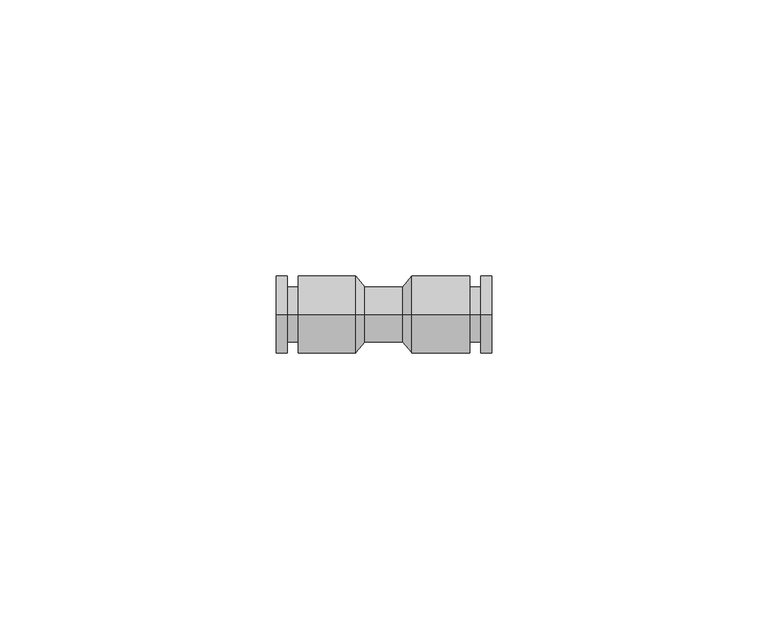
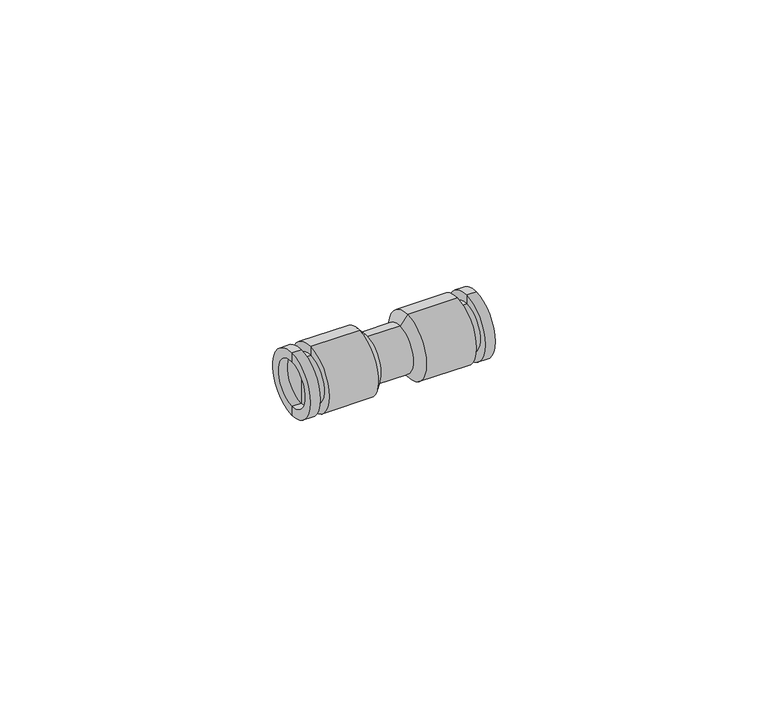
"""IFC4 building model written with IfcOpenShell, lengths in millimetres: proxy geometry, ➾ Фитинг прямой : ➾ Фитинг прямой."""

from ifc_helpers import new_model, si_unit, frame, origin, place, context, project, spatial, polyline, circle_curve, source, transform, mapped, element, save
from ifc_brep_helpers import plane_surface, cylinder_surface, revolved_surface, advanced_brep


def specialty_equipment_034aae71(model_context):
    return source(origin(), model_context, "Body", "AdvancedBrep", [
        advanced_brep(
        [(2.0, 0.0, -5.0), (2.0, 0.0, 5.0), (3.9823242, 0.0, 5.0), (3.9823242, 0.0, -5.0), (2.0, 0.0, 0.0), (37.0, 0.0, -5.0), (37.0, 0.0, 5.0), (37.0, 0.0, 0.0), (35.0176758, 0.0, -5.0), (35.0176758, 0.0, 5.0), (35.0176758, 0.0, -6.9783313), (35.0176758, 0.0, 6.9783313), (24.5665024, 0.0, -6.9783313), (24.5665024, 0.0, 6.9783313), (22.9064853, 0.0, -5.0), (22.9064853, 0.0, 5.0), (16.034289, 0.0, -5.0), (16.034289, 0.0, 5.0), (14.3742719, 0.0, -6.9783313), (14.3742719, 0.0, 6.9783313), (3.9823242, 0.0, -6.9783313), (3.9823242, 0.0, 6.9783313)],
        [
            (0, 1, circle_curve(frame((2.0, 0.0, 0.0), z_axis=(1.0, 0.0, 0.0), x_axis=(0.0, 0.0, 1.0)), 5.0)),
            (1, 2),
            (2, 3, circle_curve(frame((3.9823242, 0.0, 0.0), z_axis=(-1.0, 0.0, 0.0), x_axis=(0.0, 0.0, 1.0)), 5.0)),
            (3, 0),
            (1, 0, circle_curve(frame((2.0, 0.0, 0.0), z_axis=(1.0, 0.0, 0.0), x_axis=(0.0, 0.0, 1.0)), 5.0)),
            (3, 2, circle_curve(frame((3.9823242, 0.0, 0.0), z_axis=(-1.0, 0.0, 0.0), x_axis=(0.0, 0.0, 1.0)), 5.0)),
            (4, 1),
            (0, 4),
            (5, 6, circle_curve(frame((37.0, 0.0, 0.0), z_axis=(1.0, 0.0, 0.0), x_axis=(0.0, 0.0, 1.0)), 5.0)),
            (6, 7),
            (7, 5),
            (6, 5, circle_curve(frame((37.0, 0.0, 0.0), z_axis=(1.0, 0.0, 0.0), x_axis=(0.0, 0.0, 1.0)), 5.0)),
            (8, 9, circle_curve(frame((35.0176758, 0.0, 0.0), z_axis=(1.0, 0.0, 0.0), x_axis=(0.0, 0.0, 1.0)), 5.0)),
            (9, 6),
            (5, 8),
            (9, 8, circle_curve(frame((35.0176758, 0.0, 0.0), z_axis=(1.0, 0.0, 0.0), x_axis=(0.0, 0.0, 1.0)), 5.0)),
            (10, 11, circle_curve(frame((35.0176758, 0.0, 0.0), z_axis=(1.0, 0.0, 0.0), x_axis=(0.0, 0.0, 1.0)), 6.9783313)),
            (11, 9),
            (8, 10),
            (11, 10, circle_curve(frame((35.0176758, 0.0, 0.0), z_axis=(1.0, 0.0, 0.0), x_axis=(0.0, 0.0, 1.0)), 6.9783313)),
            (12, 13, circle_curve(frame((24.5665024, 0.0, 0.0), z_axis=(1.0, 0.0, 0.0), x_axis=(0.0, 0.0, 1.0)), 6.9783313)),
            (13, 11),
            (10, 12),
            (13, 12, circle_curve(frame((24.5665024, 0.0, 0.0), z_axis=(1.0, 0.0, 0.0), x_axis=(0.0, 0.0, 1.0)), 6.9783313)),
            (14, 15, circle_curve(frame((22.9064853, 0.0, 0.0), z_axis=(1.0, 0.0, 0.0), x_axis=(0.0, 0.0, 1.0)), 5.0)),
            (15, 13),
            (12, 14),
            (15, 14, circle_curve(frame((22.9064853, 0.0, 0.0), z_axis=(1.0, 0.0, 0.0), x_axis=(0.0, 0.0, 1.0)), 5.0)),
            (16, 17, circle_curve(frame((16.034289, 0.0, 0.0), z_axis=(1.0, 0.0, 0.0), x_axis=(0.0, 0.0, 1.0)), 5.0)),
            (17, 15),
            (14, 16),
            (17, 16, circle_curve(frame((16.034289, 0.0, 0.0), z_axis=(1.0, 0.0, 0.0), x_axis=(0.0, 0.0, 1.0)), 5.0)),
            (18, 19, circle_curve(frame((14.3742719, 0.0, 0.0), z_axis=(1.0, 0.0, 0.0), x_axis=(0.0, 0.0, 1.0)), 6.9783313)),
            (19, 17),
            (16, 18),
            (19, 18, circle_curve(frame((14.3742719, 0.0, 0.0), z_axis=(1.0, 0.0, 0.0), x_axis=(0.0, 0.0, 1.0)), 6.9783313)),
            (20, 21, circle_curve(frame((3.9823242, 0.0, 0.0), z_axis=(1.0, 0.0, 0.0), x_axis=(0.0, 0.0, 1.0)), 6.9783313)),
            (21, 19),
            (18, 20),
            (21, 20, circle_curve(frame((3.9823242, 0.0, 0.0), z_axis=(1.0, 0.0, 0.0), x_axis=(0.0, 0.0, 1.0)), 6.9783313)),
            (2, 21),
            (20, 3),
        ],
        [
            cylinder_surface(frame((-1506.5299635, 0.0, 0.0), z_axis=(-1.0, 0.0, 0.0), x_axis=(0.0, 0.0, 1.0)), 5.0),
            plane_surface(frame((2.0, 0.0, 0.0), z_axis=(-1.0, 0.0, 0.0), x_axis=(0.0, 0.0, 1.0))),
            plane_surface(frame((37.0, 0.0, 0.0), z_axis=(1.0, 0.0, 0.0), x_axis=(0.0, 0.0, 1.0))),
            plane_surface(frame((35.0176758, 0.0, 0.0), z_axis=(1.0, 0.0, 0.0), x_axis=(0.0, 0.0, 1.0))),
            cylinder_surface(frame((-1506.5299635, 0.0, 0.0), z_axis=(-1.0, 0.0, 0.0), x_axis=(0.0, 0.0, 1.0)), 6.9783313),
            revolved_surface(polyline([(24.5665024, 0.0, 6.9783313), (22.9064853, 0.0, 5.0)]), (-1506.5299635, 0.0, 0.0), (-1.0, 0.0, 0.0)),
            revolved_surface(polyline([(16.034289, 0.0, 5.0), (14.3742719, 0.0, 6.9783313)]), (-1506.5299635, 0.0, 0.0), (-1.0, 0.0, 0.0)),
            plane_surface(frame((3.9823242, 0.0, 0.0), z_axis=(-1.0, 0.0, 0.0), x_axis=(0.0, 0.0, 1.0))),
        ],
        [
            (0, [[1, 2, 3, 4]]),
            (0, [[5, -4, 6, -2]]),
            (1, [[7, -1, 8]]),
            (1, [[-8, -5, -7]]),
            (2, [[9, 10, 11]]),
            (2, [[12, -11, -10]]),
            (0, [[13, 14, -9, 15]]),
            (0, [[16, -15, -12, -14]]),
            (3, [[17, 18, -13, 19]]),
            (3, [[20, -19, -16, -18]]),
            (4, [[21, 22, -17, 23]]),
            (4, [[24, -23, -20, -22]]),
            (5, [[25, 26, -21, 27]]),
            (5, [[28, -27, -24, -26]]),
            (0, [[29, 30, -25, 31]]),
            (0, [[32, -31, -28, -30]]),
            (6, [[33, 34, -29, 35]]),
            (6, [[36, -35, -32, -34]]),
            (4, [[37, 38, -33, 39]]),
            (4, [[40, -39, -36, -38]]),
            (7, [[-3, 41, -37, 42]]),
            (7, [[-6, -42, -40, -41]]),
        ],
    ),
        advanced_brep(
        [(39.0, 0.0, -6.9783313), (39.0, 0.0, 6.9783313), (39.0, 0.0, 5.0), (39.0, 0.0, -5.0), (37.0, 0.0, -6.9783313), (37.0, 0.0, 6.9783313), (37.0, 0.0, -5.0), (37.0, 0.0, 5.0)],
        [
            (0, 1, circle_curve(frame((39.0, 0.0, 0.0), z_axis=(1.0, 0.0, 0.0), x_axis=(0.0, 0.0, 1.0)), 6.9783313)),
            (1, 2),
            (2, 3, circle_curve(frame((39.0, 0.0, 0.0), z_axis=(-1.0, 0.0, 0.0), x_axis=(0.0, 0.0, 1.0)), 5.0)),
            (3, 0),
            (1, 0, circle_curve(frame((39.0, 0.0, 0.0), z_axis=(1.0, 0.0, 0.0), x_axis=(0.0, 0.0, 1.0)), 6.9783313)),
            (3, 2, circle_curve(frame((39.0, 0.0, 0.0), z_axis=(-1.0, 0.0, 0.0), x_axis=(0.0, 0.0, 1.0)), 5.0)),
            (4, 5, circle_curve(frame((37.0, 0.0, 0.0), z_axis=(1.0, 0.0, 0.0), x_axis=(0.0, 0.0, 1.0)), 6.9783313)),
            (5, 1),
            (0, 4),
            (5, 4, circle_curve(frame((37.0, 0.0, 0.0), z_axis=(1.0, 0.0, 0.0), x_axis=(0.0, 0.0, 1.0)), 6.9783313)),
            (6, 7, circle_curve(frame((37.0, 0.0, 0.0), z_axis=(1.0, 0.0, 0.0), x_axis=(0.0, 0.0, 1.0)), 5.0)),
            (7, 5),
            (4, 6),
            (7, 6, circle_curve(frame((37.0, 0.0, 0.0), z_axis=(1.0, 0.0, 0.0), x_axis=(0.0, 0.0, 1.0)), 5.0)),
            (2, 7),
            (6, 3),
        ],
        [
            plane_surface(frame((39.0, 0.0, 0.0), z_axis=(1.0, 0.0, 0.0), x_axis=(0.0, 0.0, 1.0))),
            cylinder_surface(frame((-1469.5299635, 0.0, 0.0), z_axis=(-1.0, 0.0, 0.0), x_axis=(0.0, 0.0, 1.0)), 6.9783313),
            plane_surface(frame((37.0, 0.0, 0.0), z_axis=(-1.0, 0.0, 0.0), x_axis=(0.0, 0.0, 1.0))),
            revolved_surface(polyline([(37.0, 0.0, 5.0), (39.0, 0.0, 5.0)]), (-1469.5299635, 0.0, 0.0), (-1.0, 0.0, 0.0)),
        ],
        [
            (0, [[1, 2, 3, 4]]),
            (0, [[5, -4, 6, -2]]),
            (1, [[7, 8, -1, 9]]),
            (1, [[10, -9, -5, -8]]),
            (2, [[11, 12, -7, 13]]),
            (2, [[14, -13, -10, -12]]),
            (3, [[-3, 15, -11, 16]]),
            (3, [[-6, -16, -14, -15]]),
        ],
    ),
        advanced_brep(
        [(2.0, 0.0, -6.9783313), (2.0, 0.0, 6.9783313), (2.0, 0.0, 5.0), (2.0, 0.0, -5.0), (0.0, 0.0, -6.9783313), (0.0, 0.0, 6.9783313), (0.0, 0.0, -5.0), (0.0, 0.0, 5.0)],
        [
            (0, 1, circle_curve(frame((2.0, 0.0, 0.0), z_axis=(1.0, 0.0, 0.0), x_axis=(0.0, 0.0, 1.0)), 6.9783313)),
            (1, 2),
            (2, 3, circle_curve(frame((2.0, 0.0, 0.0), z_axis=(-1.0, 0.0, 0.0), x_axis=(0.0, 0.0, 1.0)), 5.0)),
            (3, 0),
            (1, 0, circle_curve(frame((2.0, 0.0, 0.0), z_axis=(1.0, 0.0, 0.0), x_axis=(0.0, 0.0, 1.0)), 6.9783313)),
            (3, 2, circle_curve(frame((2.0, 0.0, 0.0), z_axis=(-1.0, 0.0, 0.0), x_axis=(0.0, 0.0, 1.0)), 5.0)),
            (4, 5, circle_curve(frame((0.0, 0.0, 0.0), z_axis=(1.0, 0.0, 0.0), x_axis=(0.0, 0.0, 1.0)), 6.9783313)),
            (5, 1),
            (0, 4),
            (5, 4, circle_curve(frame((0.0, 0.0, 0.0), z_axis=(1.0, 0.0, 0.0), x_axis=(0.0, 0.0, 1.0)), 6.9783313)),
            (6, 7, circle_curve(frame((0.0, 0.0, 0.0), z_axis=(1.0, 0.0, 0.0), x_axis=(0.0, 0.0, 1.0)), 5.0)),
            (7, 5),
            (4, 6),
            (7, 6, circle_curve(frame((0.0, 0.0, 0.0), z_axis=(1.0, 0.0, 0.0), x_axis=(0.0, 0.0, 1.0)), 5.0)),
            (2, 7),
            (6, 3),
        ],
        [
            plane_surface(frame((2.0, 0.0, 0.0), z_axis=(1.0, 0.0, 0.0), x_axis=(0.0, 0.0, 1.0))),
            cylinder_surface(frame((-1506.5299635, 0.0, 0.0), z_axis=(-1.0, 0.0, 0.0), x_axis=(0.0, 0.0, 1.0)), 6.9783313),
            plane_surface(frame((0.0, 0.0, 0.0), z_axis=(-1.0, 0.0, 0.0), x_axis=(0.0, 0.0, 1.0))),
            revolved_surface(polyline([(0.0, 0.0, 5.0), (2.0, 0.0, 5.0)]), (-1506.5299635, 0.0, 0.0), (-1.0, 0.0, 0.0)),
        ],
        [
            (0, [[1, 2, 3, 4]]),
            (0, [[5, -4, 6, -2]]),
            (1, [[7, 8, -1, 9]]),
            (1, [[10, -9, -5, -8]]),
            (2, [[11, 12, -7, 13]]),
            (2, [[14, -13, -10, -12]]),
            (3, [[-3, 15, -11, 16]]),
            (3, [[-6, -16, -14, -15]]),
        ],
    ),
    ])


if __name__ == "__main__":
    model = new_model("IFC4")
    model_context = context("Model", 3, world=origin())
    ifc_project = project(units=[si_unit("LENGTHUNIT", "METRE", prefix="MILLI")], contexts=[model_context])
    site = spatial("IfcSite", under=ifc_project)
    building = spatial("IfcBuilding", under=site)
    placement = place(None, origin())
    specialty_equipment_shape = specialty_equipment_034aae71(model_context)
    element("IfcBuildingElementProxy", 1, Name="➾ Фитинг прямой : ➾ Фитинг прямой", ObjectType="➾ Фитинг прямой : ➾ Фитинг прямой", at=placement, inside=building, context=model_context, shape_type="MappedRepresentation", body=[
        mapped(specialty_equipment_shape, transform((0.0, 0.0, 0.0), x_axis=(1.0, 0.0, 0.0), y_axis=(0.0, 1.0, 0.0), z_axis=(0.0, 0.0, 1.0))),
    ])
    save(model, "model.ifc")

# Revit data of these elements
# Project information
#   Вариант конструкции = "Главная модель"
#   Дата утверждения проекта = "Дата выпуска"
#   Статус проекта = "Статус проекта"
#   Заказчик = "Владелец"
#   Адрес проекта = "Укажите адрес"
#   Наименование проекта = "Наименование проекта"
# Type "➾ Фитинг прямой : ➾ Фитинг прямой"
#   Description = "Применяется для подсоединения инъекционных трубок к инъекционным штуцерам (угловым).\r\n"
#   Manufacturer = "ТехноНИКОЛЬ"
#   ADSK_Обозначение = "ТехноНИКОЛЬ"
#   ADSK_Наименование = "Фитинг соединительный прямой 10мм \r\n"
#   ADSK_Код изделия = "419391\r\n"
#   ADSK_Завод-изготовитель = "ТехноНИКОЛЬ"
#   ADSK_Единица измерения = "шт."
#   ADSK_Группирование = "Штуцеры и аксессуары"
#   ADSK_URL страницы изделия = ""
#   ADSK_URL документации изделия = ""
#   ADSK_Количество = 1
#   Материал_Окантовка = TN_ПВХ_Синий
#   Материал_Корпус = TN_ПВХ_Черный
#   Default Elevation = 0
#   URL = ""
# Element 1 (IfcBuildingElementProxy, "➾ Фитинг прямой : ➾ Фитинг прямой")
#   Materials on its faces: "TN_ПВХ_Черный", "TN_ПВХ_Синий"
# Materials
#   "TN_ПВХ_Синий": class "Типовые", colour RGB 71 166 243, transparency 0, Cost = 0
#   "TN_ПВХ_Черный": class "Типовые", colour RGB 48 48 48, transparency 0, Cost = 0
